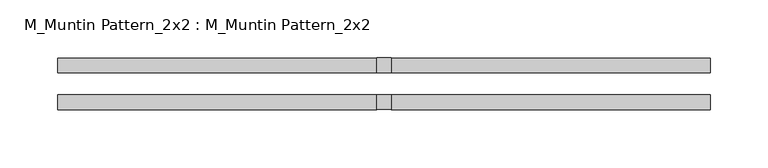
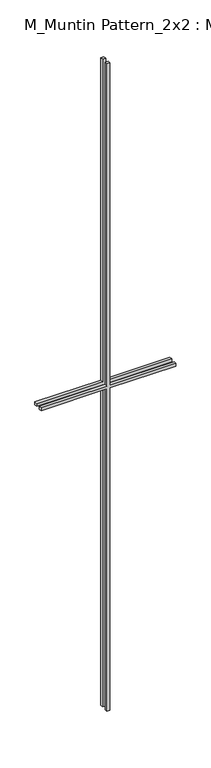
"""IFC4 building model written with IfcOpenShell, lengths in millimetres: proxy geometry, M_Muntin Pattern_2x2 : M_Muntin Pattern_2x2."""

from ifc_helpers import new_model, si_unit, frame, origin, place, context, project, spatial, polyline, outline, extrude, source, transform, mapped, element, save


def m_muntin_pattern_2x2_m_muntin_pattern_2x2_1e93d9db(model_context):
    return source(origin(), model_context, "Body", "SweptSolid", [
        extrude(outline(polyline([(1436.5, -6.35), (1436.5, -281.7375), (1423.8, -281.7375), (1423.8, -6.35), (0.0, -6.35), (0.0, 6.35), (1423.8, 6.35), (1423.8, 281.7375), (1436.5, 281.7375), (1436.5, 6.35), (2860.3, 6.35), (2860.3, -6.35), (1436.5, -6.35)])), frame((0.0, 9.525, 0.0), z_axis=(0.0, 1.0, 0.0), x_axis=(0.0, 0.0, 1.0)), (0.0, 0.0, 1.0), 12.7),
        extrude(outline(polyline([(1436.5, -6.35), (1436.5, -281.7375), (1423.8, -281.7375), (1423.8, -6.35), (0.0, -6.35), (0.0, 6.35), (1423.8, 6.35), (1423.8, 281.7375), (1436.5, 281.7375), (1436.5, 6.35), (2860.3, 6.35), (2860.3, -6.35), (1436.5, -6.35)])), frame((0.0, -22.225, 0.0), z_axis=(0.0, 1.0, 0.0), x_axis=(0.0, 0.0, 1.0)), (0.0, 0.0, 1.0), 12.7),
    ])


if __name__ == "__main__":
    model = new_model("IFC4")
    model_context = context("Model", 3, world=origin())
    ifc_project = project(units=[si_unit("LENGTHUNIT", "METRE", prefix="MILLI")], contexts=[model_context])
    site = spatial("IfcSite", under=ifc_project)
    building = spatial("IfcBuilding", under=site)
    placement = place(None, origin())
    m_muntin_pattern_2x2_m_muntin_pattern_2x2_shape = m_muntin_pattern_2x2_m_muntin_pattern_2x2_1e93d9db(model_context)
    element("IfcBuildingElementProxy", 1, Name="M_Muntin Pattern_2x2 : M_Muntin Pattern_2x2", ObjectType="M_Muntin Pattern_2x2 : M_Muntin Pattern_2x2", at=placement, inside=building, context=model_context, shape_type="MappedRepresentation", body=[
        mapped(m_muntin_pattern_2x2_m_muntin_pattern_2x2_shape, transform((0.0, 0.0, 0.0), x_axis=(1.0, 0.0, 0.0), y_axis=(0.0, 1.0, 0.0), z_axis=(0.0, 0.0, 1.0))),
    ])
    save(model, "model.ifc")

# Revit data of these elements
# Type "M_Muntin Pattern_2x2 : M_Muntin Pattern_2x2"
#   Width [instance default] = 1200 mm
#   Thickness = 12.7 mm
#   Height [instance default] = 1200 mm
#   Distance = 19.05 mm
#   Interior Material [instance default] = none
#   Exterior Material [instance default] = none
#   Default Elevation = 0
# Element 1 (IfcBuildingElementProxy, "M_Muntin Pattern_2x2 : M_Muntin Pattern_2x2")
#   Width = 563.475 mm
#   Height = 2860.3 mm
#   Interior Material = Wood - Stained
#   Exterior Material = Clad - White
#   Materials on its faces: "Clad - White", "Wood - Stained"
# Materials
#   "Clad - White": class "Wood", colour RGB 245 245 243, transparency 0, Cost = 0
#   "Wood - Stained": class "Wood", colour RGB 173 132 96, transparency 0, Cost = 0
